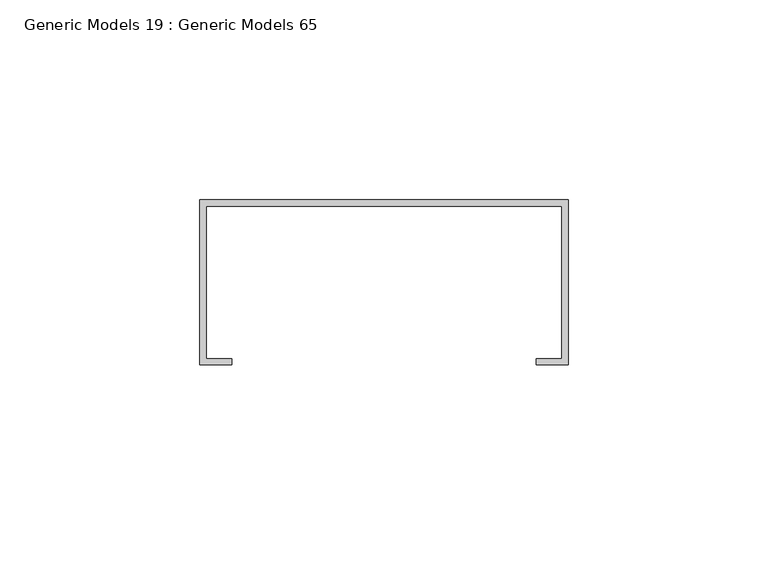
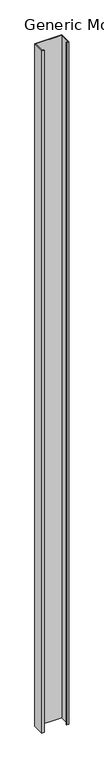
"""IFC4 building model written with IfcOpenShell, lengths in millimetres: proxy geometry, Generic Models 19 : Generic Models 65."""

import ifcopenshell
import ifcopenshell.guid

model = None  # the IFC model being written
_history = None  # IfcOwnerHistory: only IFC2X3 demands one
_inside = {}  # id of a spatial element -> (the spatial element, [elements in it])
_under = {}  # id of a project, library or spatial element -> (it, [spatial elements below it])
_declared = {}  # id of a project -> (the project, [libraries it declares])
_typed = {}  # id of a type object -> (the type object, [elements of that type])
_made_of = {}  # id of a material, layer set ... -> (it, [elements and type objects made of it])


def new_model(schema):
    """Start an empty IFC model of exactly this schema.

    Asked for "IFC4X3", IfcOpenShell would pick the latest addendum, in which some entities
    have other attributes; the version numbers below select the first issue.
    IFC2X3 requires an IfcOwnerHistory on every rooted entity: one is made here for all.
    """
    global model, _history
    if schema == "IFC4X3":
        model = ifcopenshell.file(schema_version=(4, 3, 0, 0))
    else:
        model = ifcopenshell.file(schema=schema)
    _inside.clear()
    _under.clear()
    _declared.clear()
    _typed.clear()
    _made_of.clear()
    _history = None
    if model.schema == "IFC2X3":
        org = make("IfcOrganization", Name="unknown")
        user = make(
            "IfcPersonAndOrganization",
            ThePerson=make("IfcPerson", FamilyName="unknown"),
            TheOrganization=org,
        )
        app = make(
            "IfcApplication",
            ApplicationDeveloper=org,
            Version="unknown",
            ApplicationFullName="unknown",
            ApplicationIdentifier="unknown",
        )
        _history = make(
            "IfcOwnerHistory",
            OwningUser=user,
            OwningApplication=app,
            ChangeAction="ADDED",
            CreationDate=0,
        )
    return model


def make(cls, **values):
    """One entity of the class cls with the attributes given. An attribute that is None is left unset."""
    return model.create_entity(
        cls, **{name: value for name, value in values.items() if value is not None}
    )


def rooted(cls, **values):
    """An entity with a GlobalId (a new one), such as an element, a storey or a relation."""
    return make(cls, GlobalId=ifcopenshell.guid.new(), OwnerHistory=_history, **values)


def si_unit(unit_type, name, prefix=None):
    """IfcSIUnit, for example si_unit("LENGTHUNIT", "METRE", prefix="MILLI")."""
    return make("IfcSIUnit", UnitType=unit_type, Prefix=prefix, Name=name)


def assignment(units):
    """IfcUnitAssignment: the units of a project."""
    return None if units is None else make("IfcUnitAssignment", Units=units)


def point(xyz):
    """IfcCartesianPoint."""
    return None if xyz is None else make("IfcCartesianPoint", Coordinates=xyz)


def direction(xyz):
    """IfcDirection."""
    return None if xyz is None else make("IfcDirection", DirectionRatios=xyz)


def frame(location, z_axis=None, x_axis=None):
    """IfcAxis2Placement3D, a coordinate frame: its origin and axes. An axis left out is left unset."""
    return make(
        "IfcAxis2Placement3D",
        Location=point(location),
        Axis=direction(z_axis),
        RefDirection=direction(x_axis),
    )


def origin():
    """The frame at (0, 0, 0) with its axes left unset."""
    return frame((0.0, 0.0, 0.0))


def place(relative_to, where):
    """IfcLocalPlacement: puts the frame where relative to a parent placement (None: the world)."""
    return make(
        "IfcLocalPlacement", PlacementRelTo=relative_to, RelativePlacement=where
    )


def context(
    kind, dimensions, precision=None, world=None, true_north=None, identifier=None
):
    """IfcGeometricRepresentationContext, for example the 3D "Model" context."""
    return make(
        "IfcGeometricRepresentationContext",
        ContextIdentifier=identifier,
        ContextType=kind,
        CoordinateSpaceDimension=dimensions,
        Precision=precision,
        WorldCoordinateSystem=world,
        TrueNorth=true_north,
    )


def project(units=None, contexts=None):
    """IfcProject with its units and contexts."""
    return rooted(
        "IfcProject",
        Name="project",
        RepresentationContexts=contexts,
        UnitsInContext=assignment(units),
    )


def spatial(cls, under=None, at=None, **own):
    """A site, building, storey or space (cls), placed at a placement, below another one or the project."""
    s = rooted(cls, ObjectPlacement=at, **own)
    if under is not None:
        _under.setdefault(under.id(), (under, []))[1].append(s)
    return s


def polyline(points):
    """IfcPolyline through the points."""
    return make("IfcPolyline", Points=[point(p) for p in points])


def outline(outer, holes=None, kind="AREA"):
    """IfcArbitraryClosedProfileDef: a profile drawn as a closed curve; with holes, ...WithVoids."""
    if holes is None:
        return make("IfcArbitraryClosedProfileDef", ProfileType=kind, OuterCurve=outer)
    return make(
        "IfcArbitraryProfileDefWithVoids",
        ProfileType=kind,
        OuterCurve=outer,
        InnerCurves=holes,
    )


def extrude(swept, where, along, depth):
    """IfcExtrudedAreaSolid: the profile swept, set in the frame where, extruded along a direction by depth."""
    return make(
        "IfcExtrudedAreaSolid",
        SweptArea=swept,
        Position=where,
        ExtrudedDirection=direction(along),
        Depth=depth,
    )


def shape(context_of_items, identifier, shape_type, items):
    """IfcShapeRepresentation: the items that make up one representation, for example the "Body"."""
    return make(
        "IfcShapeRepresentation",
        ContextOfItems=context_of_items,
        RepresentationIdentifier=identifier,
        RepresentationType=shape_type,
        Items=items,
    )


def source(mapping_origin, context_of_items, identifier, shape_type, items):
    """IfcRepresentationMap: a shape defined once, which mapped items show again and again."""
    return make(
        "IfcRepresentationMap",
        MappingOrigin=mapping_origin,
        MappedRepresentation=shape(context_of_items, identifier, shape_type, items),
    )


def transform(
    local_origin,
    x_axis=None,
    y_axis=None,
    z_axis=None,
    scale=None,
    scale2=None,
    scale3=None,
    uniform=True,
):
    """IfcCartesianTransformationOperator3D, or its non-uniform kind. x_axis, y_axis, z_axis: its Axis1, 2, 3."""
    if uniform:
        return make(
            "IfcCartesianTransformationOperator3D",
            Axis1=direction(x_axis),
            Axis2=direction(y_axis),
            LocalOrigin=point(local_origin),
            Scale=scale,
            Axis3=direction(z_axis),
        )
    return make(
        "IfcCartesianTransformationOperator3DnonUniform",
        Axis1=direction(x_axis),
        Axis2=direction(y_axis),
        LocalOrigin=point(local_origin),
        Scale=scale,
        Axis3=direction(z_axis),
        Scale2=scale2,
        Scale3=scale3,
    )


def mapped(mapping_source, mapping_target):
    """IfcMappedItem: shows the shape of a source again, moved by a transform."""
    return make(
        "IfcMappedItem", MappingSource=mapping_source, MappingTarget=mapping_target
    )


def made_of(thing, what):
    """Note that an element or type object is made of a material, layer set ...; save() writes the relation."""
    if what is not None:
        _made_of.setdefault(what.id(), (what, []))[1].append(thing)
    return thing


def element(
    cls,
    number,
    at=None,
    inside=None,
    cuts=None,
    type_object=None,
    material=None,
    context=None,
    identifier="Body",
    shape_type=None,
    held_by="IfcProductDefinitionShape",
    body=None,
    shapes=None,
    **own,
):
    """One element of the class cls, such as IfcWall. Its Tag is "e" and its number.

    at: its placement. inside: the storey or other place that contains it. cuts: it is an
    opening in that element (IfcRelVoidsElement). A single representation is given by context,
    identifier, shape_type and body (its items); several are given by shapes. held_by: the class
    of the entity that holds the representations. save() writes the other relations.
    """
    e = rooted(cls, Tag="e%d" % number, ObjectPlacement=at, **own)
    if body is not None:
        shapes = [shape(context, identifier, shape_type, body)]
    if shapes is not None:
        e.Representation = make(held_by, Representations=shapes)
    if inside is not None:
        _inside.setdefault(inside.id(), (inside, []))[1].append(e)
    if cuts is not None:
        rooted(
            "IfcRelVoidsElement", RelatingBuildingElement=cuts, RelatedOpeningElement=e
        )
    if type_object is not None:
        _typed.setdefault(type_object.id(), (type_object, []))[1].append(e)
    return made_of(e, material)


def aggregate(whole, parts):
    """IfcRelAggregates: a whole, such as a stair, and the parts it consists of."""
    return rooted("IfcRelAggregates", RelatingObject=whole, RelatedObjects=parts)


def save(model, path):
    """Write the relations noted so far, then the file.

    IfcRelAggregates (storeys below a building ...), IfcRelContainedInSpatialStructure (elements
    in a storey), IfcRelDefinesByType, IfcRelAssociatesMaterial and IfcRelDeclares: one each for
    every whole, place, type object, material and project.
    """
    for whole, parts in _under.values():
        aggregate(whole, parts)
    for where, things in _inside.values():
        rooted(
            "IfcRelContainedInSpatialStructure",
            RelatedElements=things,
            RelatingStructure=where,
        )
    for kind, things in _typed.values():
        rooted("IfcRelDefinesByType", RelatedObjects=things, RelatingType=kind)
    for what, things in _made_of.values():
        rooted("IfcRelAssociatesMaterial", RelatedObjects=things, RelatingMaterial=what)
    for by, libraries in _declared.values():
        rooted("IfcRelDeclares", RelatingContext=by, RelatedDefinitions=libraries)
    model.write(path)


def generic_models_19_generic_models_65_4a0df7f0(model_context):
    return source(origin(), model_context, "Body", "SweptSolid", [
        extrude(outline(polyline([(49691.925, 630.2375), (49784.0, 630.2375), (49784.0, 588.9625), (49776.0625, 588.9625), (49776.0625, 590.55), (49782.4125, 590.55), (49782.4125, 628.65), (49693.5125, 628.65), (49693.5125, 590.55), (49699.8625, 590.55), (49699.8625, 588.9625), (49691.925, 588.9625), (49691.925, 630.2375)])), frame((0.0, 0.0, 1.5875), z_axis=(0.0, 0.0, 1.0), x_axis=(1.0, 0.0, 0.0)), (0.0, 0.0, 1.0), 2454.275),
    ])


if __name__ == "__main__":
    model = new_model("IFC4")
    model_context = context("Model", 3, world=origin())
    ifc_project = project(units=[si_unit("LENGTHUNIT", "METRE", prefix="MILLI")], contexts=[model_context])
    site = spatial("IfcSite", under=ifc_project)
    building = spatial("IfcBuilding", under=site)
    placement = place(None, origin())
    generic_models_19_generic_models_65_shape = generic_models_19_generic_models_65_4a0df7f0(model_context)
    element("IfcBuildingElementProxy", 1, Name="Generic Models 19 : Generic Models 65", ObjectType="Generic Models 19 : Generic Models 65", at=placement, inside=building, context=model_context, shape_type="MappedRepresentation", body=[
        mapped(generic_models_19_generic_models_65_shape, transform((0.0, 0.0, 0.0), x_axis=(1.0, 0.0, 0.0), y_axis=(0.0, 1.0, 0.0), z_axis=(0.0, 0.0, 1.0))),
    ])
    save(model, "model.ifc")

# Revit data of these elements
# Element 1 (IfcBuildingElementProxy, "Generic Models 19 : Generic Models 65")
#   Materials on its faces: "METAL STUDS - SEE 'WALL TAG' & 'LAYER MATERIAL SCHEDULE' FOR GAUGE/SPACING & INSULATION TREATMENT, IF APPLICABLE"
# Materials
#   "METAL STUDS - SEE 'WALL TAG' & 'LAYER MATERIAL SCHEDULE' FOR GAUGE/SPACING & INSULATION TREATMENT, IF APPLICABLE": class "Unassigned", colour RGB 210 209 208, transparency 0, Keynote = "M05121300.02", Cost = 0
